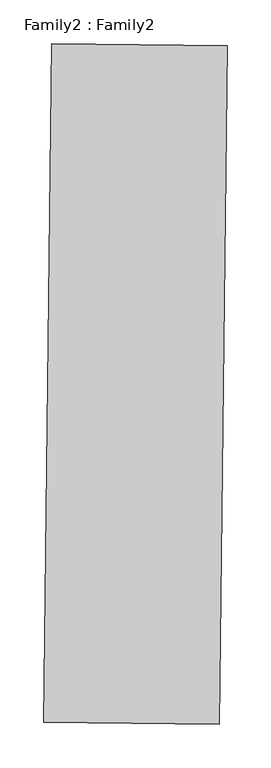
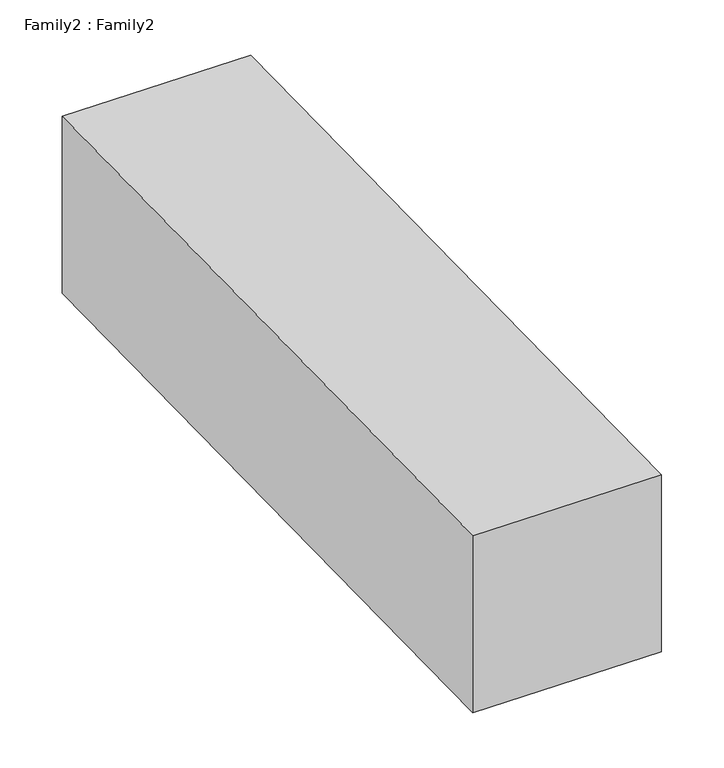
"""IFC4 building model written with IfcOpenShell, lengths in millimetres: proxy geometry, Family2 : Family2."""

import ifcopenshell
import ifcopenshell.guid

model = None  # the IFC model being written
_history = None  # IfcOwnerHistory: only IFC2X3 demands one
_inside = {}  # id of a spatial element -> (the spatial element, [elements in it])
_under = {}  # id of a project, library or spatial element -> (it, [spatial elements below it])
_declared = {}  # id of a project -> (the project, [libraries it declares])
_typed = {}  # id of a type object -> (the type object, [elements of that type])
_made_of = {}  # id of a material, layer set ... -> (it, [elements and type objects made of it])


def new_model(schema):
    """Start an empty IFC model of exactly this schema.

    Asked for "IFC4X3", IfcOpenShell would pick the latest addendum, in which some entities
    have other attributes; the version numbers below select the first issue.
    IFC2X3 requires an IfcOwnerHistory on every rooted entity: one is made here for all.
    """
    global model, _history
    if schema == "IFC4X3":
        model = ifcopenshell.file(schema_version=(4, 3, 0, 0))
    else:
        model = ifcopenshell.file(schema=schema)
    _inside.clear()
    _under.clear()
    _declared.clear()
    _typed.clear()
    _made_of.clear()
    _history = None
    if model.schema == "IFC2X3":
        org = make("IfcOrganization", Name="unknown")
        user = make(
            "IfcPersonAndOrganization",
            ThePerson=make("IfcPerson", FamilyName="unknown"),
            TheOrganization=org,
        )
        app = make(
            "IfcApplication",
            ApplicationDeveloper=org,
            Version="unknown",
            ApplicationFullName="unknown",
            ApplicationIdentifier="unknown",
        )
        _history = make(
            "IfcOwnerHistory",
            OwningUser=user,
            OwningApplication=app,
            ChangeAction="ADDED",
            CreationDate=0,
        )
    return model


def make(cls, **values):
    """One entity of the class cls with the attributes given. An attribute that is None is left unset."""
    return model.create_entity(
        cls, **{name: value for name, value in values.items() if value is not None}
    )


def rooted(cls, **values):
    """An entity with a GlobalId (a new one), such as an element, a storey or a relation."""
    return make(cls, GlobalId=ifcopenshell.guid.new(), OwnerHistory=_history, **values)


def si_unit(unit_type, name, prefix=None):
    """IfcSIUnit, for example si_unit("LENGTHUNIT", "METRE", prefix="MILLI")."""
    return make("IfcSIUnit", UnitType=unit_type, Prefix=prefix, Name=name)


def assignment(units):
    """IfcUnitAssignment: the units of a project."""
    return None if units is None else make("IfcUnitAssignment", Units=units)


def point(xyz):
    """IfcCartesianPoint."""
    return None if xyz is None else make("IfcCartesianPoint", Coordinates=xyz)


def direction(xyz):
    """IfcDirection."""
    return None if xyz is None else make("IfcDirection", DirectionRatios=xyz)


def frame(location, z_axis=None, x_axis=None):
    """IfcAxis2Placement3D, a coordinate frame: its origin and axes. An axis left out is left unset."""
    return make(
        "IfcAxis2Placement3D",
        Location=point(location),
        Axis=direction(z_axis),
        RefDirection=direction(x_axis),
    )


def origin():
    """The frame at (0, 0, 0) with its axes left unset."""
    return frame((0.0, 0.0, 0.0))


def place(relative_to, where):
    """IfcLocalPlacement: puts the frame where relative to a parent placement (None: the world)."""
    return make(
        "IfcLocalPlacement", PlacementRelTo=relative_to, RelativePlacement=where
    )


def context(
    kind, dimensions, precision=None, world=None, true_north=None, identifier=None
):
    """IfcGeometricRepresentationContext, for example the 3D "Model" context."""
    return make(
        "IfcGeometricRepresentationContext",
        ContextIdentifier=identifier,
        ContextType=kind,
        CoordinateSpaceDimension=dimensions,
        Precision=precision,
        WorldCoordinateSystem=world,
        TrueNorth=true_north,
    )


def project(units=None, contexts=None):
    """IfcProject with its units and contexts."""
    return rooted(
        "IfcProject",
        Name="project",
        RepresentationContexts=contexts,
        UnitsInContext=assignment(units),
    )


def spatial(cls, under=None, at=None, **own):
    """A site, building, storey or space (cls), placed at a placement, below another one or the project."""
    s = rooted(cls, ObjectPlacement=at, **own)
    if under is not None:
        _under.setdefault(under.id(), (under, []))[1].append(s)
    return s


def faces_of(points, faces, orient=None, outer=None):
    """IfcFace entities. A face is a list of loops; a loop is a list of indices into points, from 0.

    orient and outer hold one flag for each loop. By default every Orientation is true, the
    first loop of a face is its IfcFaceOuterBound and the others are IfcFaceBound.
    """
    made = []
    for i, loops in enumerate(faces):
        bounds = []
        for j, loop in enumerate(loops):
            is_outer = j == 0 if outer is None else outer[i][j]
            bounds.append(
                make(
                    "IfcFaceOuterBound" if is_outer else "IfcFaceBound",
                    Bound=make("IfcPolyLoop", Polygon=[points[k] for k in loop]),
                    Orientation=True if orient is None else orient[i][j],
                )
            )
        made.append(make("IfcFace", Bounds=bounds))
    return made


def faceted_brep(points, faces, orient=None, outer=None, voids=None):
    """IfcFacetedBrep: a solid bounded by flat faces; with voids (closed shells), ...WithVoids."""
    shared = [point(p) for p in points]
    hull = make("IfcClosedShell", CfsFaces=faces_of(shared, faces, orient, outer))
    if voids is None:
        return make("IfcFacetedBrep", Outer=hull)
    return make(
        "IfcFacetedBrepWithVoids",
        Outer=hull,
        Voids=[
            make(cls, CfsFaces=faces_of(shared, fs, o, b)) for cls, fs, o, b in voids
        ],
    )


def shape(context_of_items, identifier, shape_type, items):
    """IfcShapeRepresentation: the items that make up one representation, for example the "Body"."""
    return make(
        "IfcShapeRepresentation",
        ContextOfItems=context_of_items,
        RepresentationIdentifier=identifier,
        RepresentationType=shape_type,
        Items=items,
    )


def source(mapping_origin, context_of_items, identifier, shape_type, items):
    """IfcRepresentationMap: a shape defined once, which mapped items show again and again."""
    return make(
        "IfcRepresentationMap",
        MappingOrigin=mapping_origin,
        MappedRepresentation=shape(context_of_items, identifier, shape_type, items),
    )


def transform(
    local_origin,
    x_axis=None,
    y_axis=None,
    z_axis=None,
    scale=None,
    scale2=None,
    scale3=None,
    uniform=True,
):
    """IfcCartesianTransformationOperator3D, or its non-uniform kind. x_axis, y_axis, z_axis: its Axis1, 2, 3."""
    if uniform:
        return make(
            "IfcCartesianTransformationOperator3D",
            Axis1=direction(x_axis),
            Axis2=direction(y_axis),
            LocalOrigin=point(local_origin),
            Scale=scale,
            Axis3=direction(z_axis),
        )
    return make(
        "IfcCartesianTransformationOperator3DnonUniform",
        Axis1=direction(x_axis),
        Axis2=direction(y_axis),
        LocalOrigin=point(local_origin),
        Scale=scale,
        Axis3=direction(z_axis),
        Scale2=scale2,
        Scale3=scale3,
    )


def mapped(mapping_source, mapping_target):
    """IfcMappedItem: shows the shape of a source again, moved by a transform."""
    return make(
        "IfcMappedItem", MappingSource=mapping_source, MappingTarget=mapping_target
    )


def made_of(thing, what):
    """Note that an element or type object is made of a material, layer set ...; save() writes the relation."""
    if what is not None:
        _made_of.setdefault(what.id(), (what, []))[1].append(thing)
    return thing


def element(
    cls,
    number,
    at=None,
    inside=None,
    cuts=None,
    type_object=None,
    material=None,
    context=None,
    identifier="Body",
    shape_type=None,
    held_by="IfcProductDefinitionShape",
    body=None,
    shapes=None,
    **own,
):
    """One element of the class cls, such as IfcWall. Its Tag is "e" and its number.

    at: its placement. inside: the storey or other place that contains it. cuts: it is an
    opening in that element (IfcRelVoidsElement). A single representation is given by context,
    identifier, shape_type and body (its items); several are given by shapes. held_by: the class
    of the entity that holds the representations. save() writes the other relations.
    """
    e = rooted(cls, Tag="e%d" % number, ObjectPlacement=at, **own)
    if body is not None:
        shapes = [shape(context, identifier, shape_type, body)]
    if shapes is not None:
        e.Representation = make(held_by, Representations=shapes)
    if inside is not None:
        _inside.setdefault(inside.id(), (inside, []))[1].append(e)
    if cuts is not None:
        rooted(
            "IfcRelVoidsElement", RelatingBuildingElement=cuts, RelatedOpeningElement=e
        )
    if type_object is not None:
        _typed.setdefault(type_object.id(), (type_object, []))[1].append(e)
    return made_of(e, material)


def aggregate(whole, parts):
    """IfcRelAggregates: a whole, such as a stair, and the parts it consists of."""
    return rooted("IfcRelAggregates", RelatingObject=whole, RelatedObjects=parts)


def save(model, path):
    """Write the relations noted so far, then the file.

    IfcRelAggregates (storeys below a building ...), IfcRelContainedInSpatialStructure (elements
    in a storey), IfcRelDefinesByType, IfcRelAssociatesMaterial and IfcRelDeclares: one each for
    every whole, place, type object, material and project.
    """
    for whole, parts in _under.values():
        aggregate(whole, parts)
    for where, things in _inside.values():
        rooted(
            "IfcRelContainedInSpatialStructure",
            RelatedElements=things,
            RelatingStructure=where,
        )
    for kind, things in _typed.values():
        rooted("IfcRelDefinesByType", RelatedObjects=things, RelatingType=kind)
    for what, things in _made_of.values():
        rooted("IfcRelAssociatesMaterial", RelatedObjects=things, RelatingMaterial=what)
    for by, libraries in _declared.values():
        rooted("IfcRelDeclares", RelatingContext=by, RelatedDefinitions=libraries)
    model.write(path)


def family2_family2_1a1626fa(model_context):
    return source(origin(), model_context, "Body", "Brep", [
        faceted_brep([(-3947.8668207, -6460.6173325, 1.0945136), (-3947.8668207, -6460.6173325, 201.0945136), (-3938.9759738, -5686.9827901, 202.060409), (-3938.9759738, -5686.9827901, 2.060409), (-3747.8756307, -6462.4945452, 201.0945136), (-3738.9847838, -5688.8600027, 202.060409), (-3747.8756307, -6462.4945452, 1.0945136), (-3738.9847838, -5688.8600027, 2.060409)], [[[0, 1, 2, 3]], [[1, 4, 5, 2]], [[4, 6, 7, 5]], [[6, 0, 3, 7]], [[3, 2, 5, 7]], [[0, 6, 4, 1]]]),
    ])


if __name__ == "__main__":
    model = new_model("IFC4")
    model_context = context("Model", 3, world=origin())
    ifc_project = project(units=[si_unit("LENGTHUNIT", "METRE", prefix="MILLI")], contexts=[model_context])
    site = spatial("IfcSite", under=ifc_project)
    building = spatial("IfcBuilding", under=site)
    placement = place(None, origin())
    family2_family2_shape = family2_family2_1a1626fa(model_context)
    element("IfcBuildingElementProxy", 1, Name="Family2 : Family2", ObjectType="Family2 : Family2", at=placement, inside=building, context=model_context, shape_type="MappedRepresentation", body=[
        mapped(family2_family2_shape, transform((0.0, 0.0, 0.0), x_axis=(1.0, 0.0, 0.0), y_axis=(0.0, 1.0, 0.0), z_axis=(0.0, 0.0, 1.0))),
    ])
    save(model, "model.ifc")

# Revit data of these elements
# Type "Family2 : Family2"
#   Default Elevation = 0
